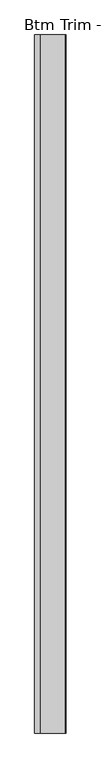
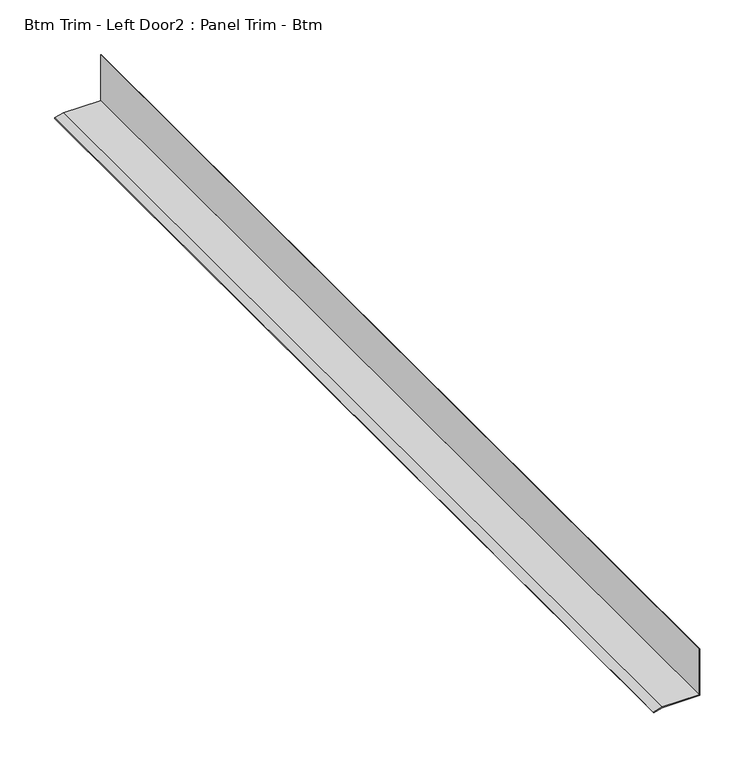
"""IFC4 building model written with IfcOpenShell, lengths in millimetres: proxy geometry, Btm Trim - Left Door2 : Panel Trim - Btm."""

from ifc_helpers import new_model, si_unit, frame, origin, place, context, project, spatial, polyline, outline, extrude, source, transform, mapped, element, save


def btm_trim_left_door2_panel_trim_btm_813b1cb6(model_context):
    return source(origin(), model_context, "Body", "SweptSolid", [
        extrude(outline(polyline([(50.8, 587326.1141748), (48.3077022, 587316.8127928), (47.5409986, 587317.0182304), (50.00625, 587326.2186739), (50.00625, 587365.8934739), (101.6, 587365.8934739), (101.6, 587365.1060739), (50.8, 587365.1060739), (50.8, 587326.1141748)])), frame((0.0, -532878.2537841, 0.0), z_axis=(0.0, 1.0, 0.0), x_axis=(0.0, 0.0, 1.0)), (0.0, 0.0, 1.0), 1093.7880247),
    ])


if __name__ == "__main__":
    model = new_model("IFC4")
    model_context = context("Model", 3, world=origin())
    ifc_project = project(units=[si_unit("LENGTHUNIT", "METRE", prefix="MILLI")], contexts=[model_context])
    site = spatial("IfcSite", under=ifc_project)
    building = spatial("IfcBuilding", under=site)
    placement = place(None, origin())
    btm_trim_left_door2_panel_trim_btm_shape = btm_trim_left_door2_panel_trim_btm_813b1cb6(model_context)
    element("IfcBuildingElementProxy", 1, Name="Btm Trim - Left Door2 : Panel Trim - Btm", ObjectType="Btm Trim - Left Door2 : Panel Trim - Btm", at=placement, inside=building, context=model_context, shape_type="MappedRepresentation", body=[
        mapped(btm_trim_left_door2_panel_trim_btm_shape, transform((0.0, 0.0, 0.0), x_axis=(1.0, 0.0, 0.0), y_axis=(0.0, 1.0, 0.0), z_axis=(0.0, 0.0, 1.0))),
    ])
    save(model, "model.ifc")

# Revit data of these elements
# Element 1 (IfcBuildingElementProxy, "Btm Trim - Left Door2 : Panel Trim - Btm")
#   Materials on its faces: "BASE TRIM BY MTL PANEL MFR."
# Materials
#   "BASE TRIM BY MTL PANEL MFR.": class "Generic", colour RGB 239 242 240, transparency 0, Cost = 0
